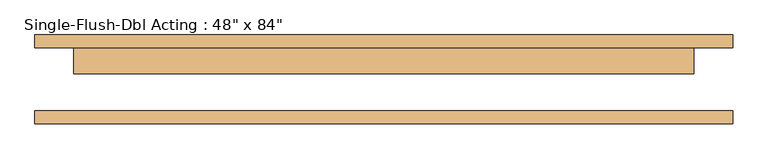
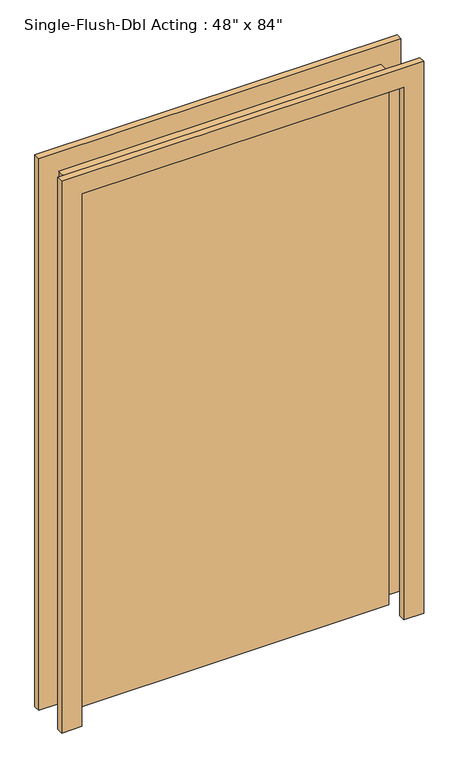
"""IFC4 building model written with IfcOpenShell, lengths in millimetres: door geometry."""

import ifcopenshell
import ifcopenshell.guid

model = None  # the IFC model being written
_history = None  # IfcOwnerHistory: only IFC2X3 demands one
_inside = {}  # id of a spatial element -> (the spatial element, [elements in it])
_under = {}  # id of a project, library or spatial element -> (it, [spatial elements below it])
_declared = {}  # id of a project -> (the project, [libraries it declares])
_typed = {}  # id of a type object -> (the type object, [elements of that type])
_made_of = {}  # id of a material, layer set ... -> (it, [elements and type objects made of it])


def new_model(schema):
    """Start an empty IFC model of exactly this schema.

    Asked for "IFC4X3", IfcOpenShell would pick the latest addendum, in which some entities
    have other attributes; the version numbers below select the first issue.
    IFC2X3 requires an IfcOwnerHistory on every rooted entity: one is made here for all.
    """
    global model, _history
    if schema == "IFC4X3":
        model = ifcopenshell.file(schema_version=(4, 3, 0, 0))
    else:
        model = ifcopenshell.file(schema=schema)
    _inside.clear()
    _under.clear()
    _declared.clear()
    _typed.clear()
    _made_of.clear()
    _history = None
    if model.schema == "IFC2X3":
        org = make("IfcOrganization", Name="unknown")
        user = make(
            "IfcPersonAndOrganization",
            ThePerson=make("IfcPerson", FamilyName="unknown"),
            TheOrganization=org,
        )
        app = make(
            "IfcApplication",
            ApplicationDeveloper=org,
            Version="unknown",
            ApplicationFullName="unknown",
            ApplicationIdentifier="unknown",
        )
        _history = make(
            "IfcOwnerHistory",
            OwningUser=user,
            OwningApplication=app,
            ChangeAction="ADDED",
            CreationDate=0,
        )
    return model


def make(cls, **values):
    """One entity of the class cls with the attributes given. An attribute that is None is left unset."""
    return model.create_entity(
        cls, **{name: value for name, value in values.items() if value is not None}
    )


def rooted(cls, **values):
    """An entity with a GlobalId (a new one), such as an element, a storey or a relation."""
    return make(cls, GlobalId=ifcopenshell.guid.new(), OwnerHistory=_history, **values)


def si_unit(unit_type, name, prefix=None):
    """IfcSIUnit, for example si_unit("LENGTHUNIT", "METRE", prefix="MILLI")."""
    return make("IfcSIUnit", UnitType=unit_type, Prefix=prefix, Name=name)


def assignment(units):
    """IfcUnitAssignment: the units of a project."""
    return None if units is None else make("IfcUnitAssignment", Units=units)


def point(xyz):
    """IfcCartesianPoint."""
    return None if xyz is None else make("IfcCartesianPoint", Coordinates=xyz)


def direction(xyz):
    """IfcDirection."""
    return None if xyz is None else make("IfcDirection", DirectionRatios=xyz)


def frame(location, z_axis=None, x_axis=None):
    """IfcAxis2Placement3D, a coordinate frame: its origin and axes. An axis left out is left unset."""
    return make(
        "IfcAxis2Placement3D",
        Location=point(location),
        Axis=direction(z_axis),
        RefDirection=direction(x_axis),
    )


def origin():
    """The frame at (0, 0, 0) with its axes left unset."""
    return frame((0.0, 0.0, 0.0))


def origin_with_axes():
    """The frame at (0, 0, 0) with the z axis (0, 0, 1) and the x axis (1, 0, 0) written out."""
    return frame((0.0, 0.0, 0.0), z_axis=(0.0, 0.0, 1.0), x_axis=(1.0, 0.0, 0.0))


def place(relative_to, where):
    """IfcLocalPlacement: puts the frame where relative to a parent placement (None: the world)."""
    return make(
        "IfcLocalPlacement", PlacementRelTo=relative_to, RelativePlacement=where
    )


def context(
    kind, dimensions, precision=None, world=None, true_north=None, identifier=None
):
    """IfcGeometricRepresentationContext, for example the 3D "Model" context."""
    return make(
        "IfcGeometricRepresentationContext",
        ContextIdentifier=identifier,
        ContextType=kind,
        CoordinateSpaceDimension=dimensions,
        Precision=precision,
        WorldCoordinateSystem=world,
        TrueNorth=true_north,
    )


def project(units=None, contexts=None):
    """IfcProject with its units and contexts."""
    return rooted(
        "IfcProject",
        Name="project",
        RepresentationContexts=contexts,
        UnitsInContext=assignment(units),
    )


def spatial(cls, under=None, at=None, **own):
    """A site, building, storey or space (cls), placed at a placement, below another one or the project."""
    s = rooted(cls, ObjectPlacement=at, **own)
    if under is not None:
        _under.setdefault(under.id(), (under, []))[1].append(s)
    return s


def polyline(points):
    """IfcPolyline through the points."""
    return make("IfcPolyline", Points=[point(p) for p in points])


def outline(outer, holes=None, kind="AREA"):
    """IfcArbitraryClosedProfileDef: a profile drawn as a closed curve; with holes, ...WithVoids."""
    if holes is None:
        return make("IfcArbitraryClosedProfileDef", ProfileType=kind, OuterCurve=outer)
    return make(
        "IfcArbitraryProfileDefWithVoids",
        ProfileType=kind,
        OuterCurve=outer,
        InnerCurves=holes,
    )


def extrude(swept, where, along, depth):
    """IfcExtrudedAreaSolid: the profile swept, set in the frame where, extruded along a direction by depth."""
    return make(
        "IfcExtrudedAreaSolid",
        SweptArea=swept,
        Position=where,
        ExtrudedDirection=direction(along),
        Depth=depth,
    )


def shape(context_of_items, identifier, shape_type, items):
    """IfcShapeRepresentation: the items that make up one representation, for example the "Body"."""
    return make(
        "IfcShapeRepresentation",
        ContextOfItems=context_of_items,
        RepresentationIdentifier=identifier,
        RepresentationType=shape_type,
        Items=items,
    )


def source(mapping_origin, context_of_items, identifier, shape_type, items):
    """IfcRepresentationMap: a shape defined once, which mapped items show again and again."""
    return make(
        "IfcRepresentationMap",
        MappingOrigin=mapping_origin,
        MappedRepresentation=shape(context_of_items, identifier, shape_type, items),
    )


def transform(
    local_origin,
    x_axis=None,
    y_axis=None,
    z_axis=None,
    scale=None,
    scale2=None,
    scale3=None,
    uniform=True,
):
    """IfcCartesianTransformationOperator3D, or its non-uniform kind. x_axis, y_axis, z_axis: its Axis1, 2, 3."""
    if uniform:
        return make(
            "IfcCartesianTransformationOperator3D",
            Axis1=direction(x_axis),
            Axis2=direction(y_axis),
            LocalOrigin=point(local_origin),
            Scale=scale,
            Axis3=direction(z_axis),
        )
    return make(
        "IfcCartesianTransformationOperator3DnonUniform",
        Axis1=direction(x_axis),
        Axis2=direction(y_axis),
        LocalOrigin=point(local_origin),
        Scale=scale,
        Axis3=direction(z_axis),
        Scale2=scale2,
        Scale3=scale3,
    )


def mapped(mapping_source, mapping_target):
    """IfcMappedItem: shows the shape of a source again, moved by a transform."""
    return make(
        "IfcMappedItem", MappingSource=mapping_source, MappingTarget=mapping_target
    )


def made_of(thing, what):
    """Note that an element or type object is made of a material, layer set ...; save() writes the relation."""
    if what is not None:
        _made_of.setdefault(what.id(), (what, []))[1].append(thing)
    return thing


def element(
    cls,
    number,
    at=None,
    inside=None,
    cuts=None,
    type_object=None,
    material=None,
    context=None,
    identifier="Body",
    shape_type=None,
    held_by="IfcProductDefinitionShape",
    body=None,
    shapes=None,
    **own,
):
    """One element of the class cls, such as IfcWall. Its Tag is "e" and its number.

    at: its placement. inside: the storey or other place that contains it. cuts: it is an
    opening in that element (IfcRelVoidsElement). A single representation is given by context,
    identifier, shape_type and body (its items); several are given by shapes. held_by: the class
    of the entity that holds the representations. save() writes the other relations.
    """
    e = rooted(cls, Tag="e%d" % number, ObjectPlacement=at, **own)
    if body is not None:
        shapes = [shape(context, identifier, shape_type, body)]
    if shapes is not None:
        e.Representation = make(held_by, Representations=shapes)
    if inside is not None:
        _inside.setdefault(inside.id(), (inside, []))[1].append(e)
    if cuts is not None:
        rooted(
            "IfcRelVoidsElement", RelatingBuildingElement=cuts, RelatedOpeningElement=e
        )
    if type_object is not None:
        _typed.setdefault(type_object.id(), (type_object, []))[1].append(e)
    return made_of(e, material)


def aggregate(whole, parts):
    """IfcRelAggregates: a whole, such as a stair, and the parts it consists of."""
    return rooted("IfcRelAggregates", RelatingObject=whole, RelatedObjects=parts)


def save(model, path):
    """Write the relations noted so far, then the file.

    IfcRelAggregates (storeys below a building ...), IfcRelContainedInSpatialStructure (elements
    in a storey), IfcRelDefinesByType, IfcRelAssociatesMaterial and IfcRelDeclares: one each for
    every whole, place, type object, material and project.
    """
    for whole, parts in _under.values():
        aggregate(whole, parts)
    for where, things in _inside.values():
        rooted(
            "IfcRelContainedInSpatialStructure",
            RelatedElements=things,
            RelatingStructure=where,
        )
    for kind, things in _typed.values():
        rooted("IfcRelDefinesByType", RelatedObjects=things, RelatingType=kind)
    for what, things in _made_of.values():
        rooted("IfcRelAssociatesMaterial", RelatedObjects=things, RelatingMaterial=what)
    for by, libraries in _declared.values():
        rooted("IfcRelDeclares", RelatingContext=by, RelatedDefinitions=libraries)
    model.write(path)


def door_0c2cb489(model_context):
    return source(origin(), model_context, "Body", "SweptSolid", [
        extrude(outline(polyline([(2209.8, -685.8), (0.0, -685.8), (0.0, -609.6), (2133.6, -609.6), (2133.6, 609.6), (0.0, 609.6), (0.0, 685.8), (2209.8, 685.8), (2209.8, -685.8)])), frame((0.0, 61.9125, 0.0), z_axis=(0.0, 1.0, 0.0), x_axis=(0.0, 0.0, 1.0)), (0.0, 0.0, 1.0), 25.4),
        extrude(outline(polyline([(2209.8, 685.8), (2209.8, -685.8), (0.0, -685.8), (0.0, -609.6), (2133.6, -609.6), (2133.6, 609.6), (0.0, 609.6), (0.0, 685.8), (2209.8, 685.8)])), frame((0.0, -87.3125, 0.0), z_axis=(0.0, 1.0, 0.0), x_axis=(0.0, 0.0, 1.0)), (0.0, 0.0, 1.0), 25.4),
        extrude(outline(polyline([(609.6, 11.1125), (-609.6, 11.1125), (-609.6, 61.9125), (609.6, 61.9125), (609.6, 11.1125)])), origin_with_axes(), (0.0, 0.0, 1.0), 2133.6),
    ])


if __name__ == "__main__":
    model = new_model("IFC4")
    model_context = context("Model", 3, world=origin())
    ifc_project = project(units=[si_unit("LENGTHUNIT", "METRE", prefix="MILLI")], contexts=[model_context])
    site = spatial("IfcSite", under=ifc_project)
    building = spatial("IfcBuilding", under=site)
    placement = place(None, origin())
    door_shape = door_0c2cb489(model_context)
    element("IfcDoor", 1, ObjectType="Single-Flush-Dbl Acting : 48\" x 84\"", at=placement, inside=building, context=model_context, shape_type="MappedRepresentation", body=[
        mapped(door_shape, transform((0.0, 0.0, 0.0), x_axis=(1.0, 0.0, 0.0), y_axis=(0.0, 1.0, 0.0), z_axis=(0.0, 0.0, 1.0))),
    ])
    save(model, "model.ifc")

# Revit data of these elements
# Project information
#   Room Abbreviation = "VS001"
#   Room Description = "Operating Room, Veterinary (VS001)"
#   Sheets - Total = "6"
#   Project Issue Date = "Issue Date"
#   Project Status = "Project Status"
#   Client Name = "Owner"
#   Project Address = "Enter address here"
#   Project Name = "Project Name"
#   Project Number = "Project Number"
#   Publication Date = "30-Jan-15"
# Type "Single-Flush-Dbl Acting : 48\" x 84\""
#   Type Mark = "23"
#   Construction Type = "H"
#   Assembly Code = "C1020"
#   Thickness = 0' - 2"
#   Height = 7' - 0"
#   Rail Width - Center = 0' - 4"
#   Trim Projection Ext. = 0' - 1"
#   Trim Projection Int. = 0' - 1"
#   Trim Width Ext. = 0' - 3"
#   Trim Width Int. = 0' - 3"
#   Width = 4' - 0"
#   Door Material = Door - Panel
#   Frame Material = Door - Frame
#   Function = (empty or 0)
#   Wall Closure = (empty or 0)
# Element 1 (IfcDoor, "Single-Flush-Dbl Acting : 48\" x 84\"")
#   Materials on its faces: "Door - Frame", "Door - Panel"
# Materials
#   "Door - Panel": class "Wood", colour RGB 210 159 95, transparency 0
#   "Door - Frame": class "Miscellaneous", colour RGB 118 70 51, transparency 0
